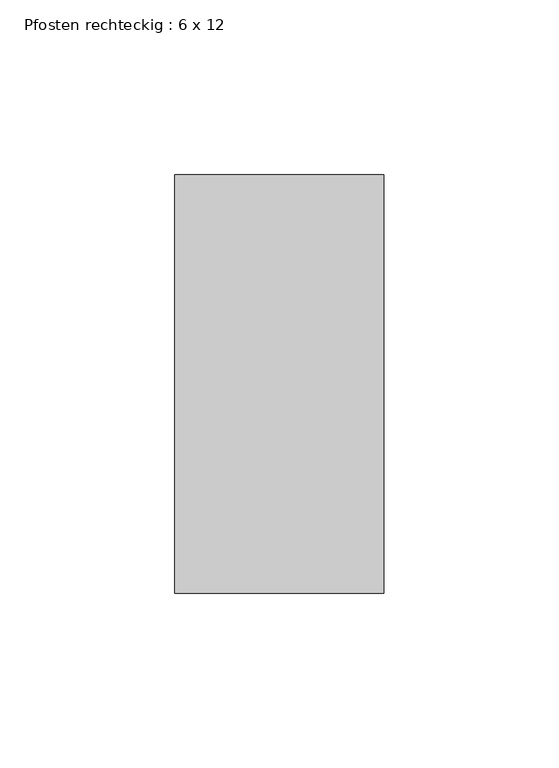
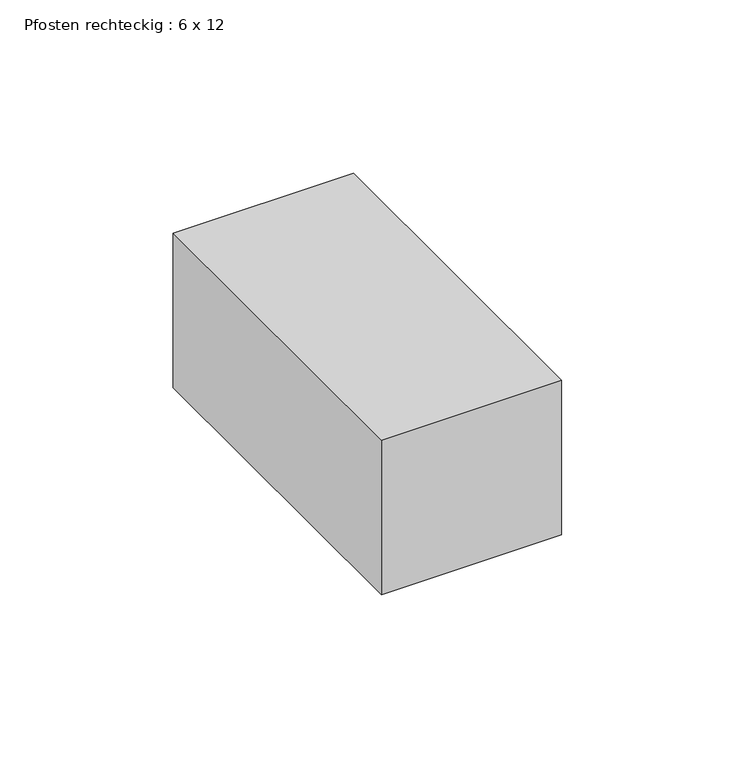
"""IFC4 building model written with IfcOpenShell, lengths in millimetres: member geometry, Pfosten rechteckig : 6 x 12."""

from ifc_helpers import new_model, si_unit, frame, origin, place, context, project, spatial, polyline, outline, extrude, source, transform, mapped, element, save


def pfosten_rechteckig_6_x_12_8f0623e0(model_context):
    return source(origin(), model_context, "Body", "SweptSolid", [
        extrude(outline(polyline([(0.0, 60.0), (0.0, -60.0), (-60.0, -60.0), (-60.0, 60.0), (0.0, 60.0)])), frame((0.0, 0.0, -54.3558419), z_axis=(0.0, 0.0, 1.0), x_axis=(1.0, 0.0, 0.0)), (0.0, 0.0, 1.0), 54.3558419),
    ])


if __name__ == "__main__":
    model = new_model("IFC4")
    model_context = context("Model", 3, world=origin())
    ifc_project = project(units=[si_unit("LENGTHUNIT", "METRE", prefix="MILLI")], contexts=[model_context])
    site = spatial("IfcSite", under=ifc_project)
    building = spatial("IfcBuilding", under=site)
    placement = place(None, origin())
    pfosten_rechteckig_6_x_12_shape = pfosten_rechteckig_6_x_12_8f0623e0(model_context)
    element("IfcMember", 1, ObjectType="Pfosten rechteckig : 6 x 12", at=placement, inside=building, context=model_context, shape_type="MappedRepresentation", body=[
        mapped(pfosten_rechteckig_6_x_12_shape, transform((0.0, 0.0, 0.0), x_axis=(1.0, 0.0, 0.0), y_axis=(0.0, 1.0, 0.0), z_axis=(0.0, 0.0, 1.0))),
    ])
    save(model, "model.ifc")

# Revit data of these elements
# Type "Pfosten rechteckig : 6 x 12"
#   built-in parameter 1007304 = 0.393701 (stored number, unit not read)
#   built-in parameter 1007301 = 0.0984252 (stored number, unit not read)
#   built-in parameter 1007300 = 0.0984252 (stored number, unit not read)
# Element 1 (IfcMember, "Pfosten rechteckig : 6 x 12")
#   Materials on its faces: "Metall - verzinkt"
# Materials
#   "Metall - verzinkt": class "Allgemeines", colour RGB 200 200 200, transparency 0, Cost = 0
